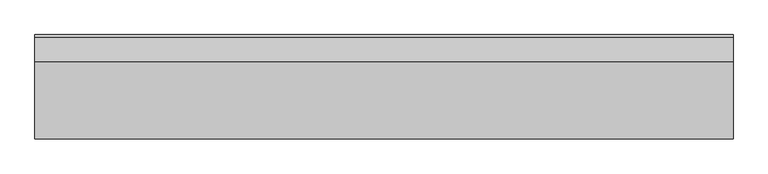
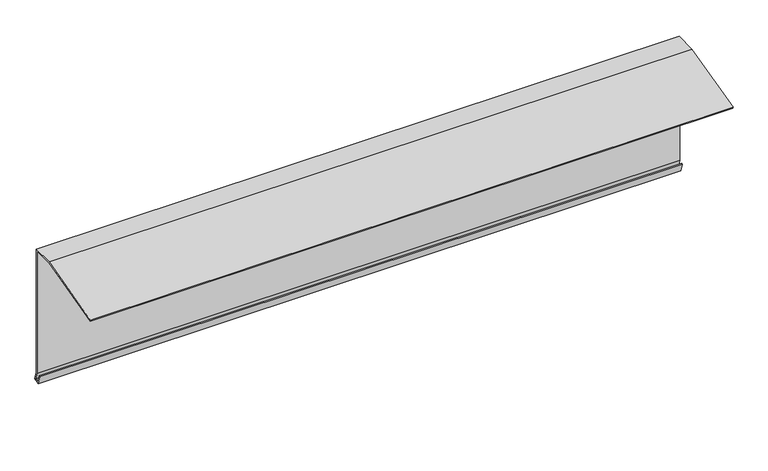
"""IFC4 building model written with IfcOpenShell, lengths in millimetres: proxy geometry, Flashing21:Flashing030:306050 : Flashing21:Flashing030:306050."""

from ifc_helpers import new_model, si_unit, frame, origin, place, context, project, spatial, polyline, outline, extrude, source, transform, mapped, element, save


def generic_models_6b814d3c(model_context):
    return source(origin(), model_context, "Body", "SweptSolid", [
        extrude(outline(polyline([(10818.1245413, 43848.4091467), (11040.1123983, 43905.1238578), (11108.9351577, 43905.1238578), (11108.9351577, 43500.7036908), (11117.2209067, 43473.7122248), (11099.6589175, 43468.3211047), (11091.1374332, 43495.8445422), (11094.9584855, 43497.0275717), (11102.3013873, 43473.3108235), (11112.2289252, 43476.3435481), (11104.9351577, 43500.1035576), (11104.9351577, 43901.1238578), (11040.6152928, 43901.1238578), (10819.11468, 43844.5336305), (10818.1245413, 43848.4091467)])), frame((8404.1994034, 0.0, 0.0), z_axis=(1.0, 0.0, 0.0), x_axis=(0.0, 1.0, 0.0)), (0.0, 0.0, 1.0), 1999.85),
    ])


if __name__ == "__main__":
    model = new_model("IFC4")
    model_context = context("Model", 3, world=origin())
    ifc_project = project(units=[si_unit("LENGTHUNIT", "METRE", prefix="MILLI")], contexts=[model_context])
    site = spatial("IfcSite", under=ifc_project)
    building = spatial("IfcBuilding", under=site)
    placement = place(None, origin())
    generic_models_shape = generic_models_6b814d3c(model_context)
    element("IfcBuildingElementProxy", 1, Name="Flashing21:Flashing030:306050 : Flashing21:Flashing030:306050", ObjectType="Flashing21:Flashing030:306050 : Flashing21:Flashing030:306050", at=placement, inside=building, context=model_context, shape_type="MappedRepresentation", body=[
        mapped(generic_models_shape, transform((0.0, 0.0, 0.0), x_axis=(1.0, 0.0, 0.0), y_axis=(0.0, 1.0, 0.0), z_axis=(0.0, 0.0, 1.0))),
    ])
    save(model, "model.ifc")

# Revit data of these elements
# Type "Flashing21:Flashing030:306050 : Flashing21:Flashing030:306050"
#   NameOverride = "Flashing21:Flashing030:306050"
#   ObjectTypeOverride = "Flashing21:Flashing030"
#   Reference = "Flashing030"
#   Category = "Generic Models"
#   Tag = "306050"
# Element 1 (IfcBuildingElementProxy, "Flashing21:Flashing030:306050 : Flashing21:Flashing030:306050")
#   Materials on its faces: "BRAKE METAL EAVE TRIM TO MATCH STANDING SEAM COLOR"
# Materials
#   "BRAKE METAL EAVE TRIM TO MATCH STANDING SEAM COLOR": class "Unassigned", colour RGB 128 128 128, transparency 0, Cost = 0
